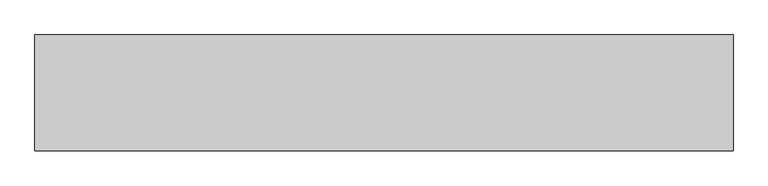
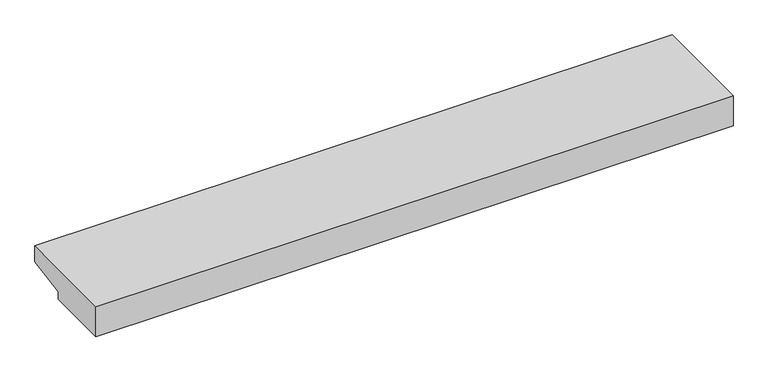
"""IFC4 building model written with IfcOpenShell, lengths in millimetres: plate geometry, 린텔1 : 창대석."""

from ifc_helpers import new_model, si_unit, frame, origin, place, context, project, spatial, polyline, outline, extrude, source, transform, mapped, element, save


def plate_352e0ffc(model_context):
    return source(origin(), model_context, "Body", "SweptSolid", [
        extrude(outline(polyline([(-195.0, 990.0), (435.0, 990.0), (435.0, 890.0), (195.0, 847.6815246), (195.0, 800.0), (-195.0, 800.0), (-195.0, 990.0)])), frame((-1900.0, 0.0, 0.0), z_axis=(1.0, 0.0, 0.0), x_axis=(0.0, 1.0, 0.0)), (0.0, 0.0, 1.0), 3800.0),
    ])


if __name__ == "__main__":
    model = new_model("IFC4")
    model_context = context("Model", 3, world=origin())
    ifc_project = project(units=[si_unit("LENGTHUNIT", "METRE", prefix="MILLI")], contexts=[model_context])
    site = spatial("IfcSite", under=ifc_project)
    building = spatial("IfcBuilding", under=site)
    placement = place(None, origin())
    plate_shape = plate_352e0ffc(model_context)
    element("IfcPlate", 1, ObjectType="린텔1 : 창대석", at=placement, inside=building, context=model_context, shape_type="MappedRepresentation", body=[
        mapped(plate_shape, transform((0.0, 0.0, 0.0), x_axis=(1.0, 0.0, 0.0), y_axis=(0.0, 1.0, 0.0), z_axis=(0.0, 0.0, 1.0))),
    ])
    save(model, "model.ifc")

# Revit data of these elements
# Type "린텔1 : 창대석"
#   Description = "THK.30 GRANITE COUNTER(TYP.)"
#   Type Mark = "200"
#   Description = "THK.30 GRANITE COUNTER(TYP.)"
#   Width = 3800 mm
#   Height = 190 mm
#   두께 = 190 mm
#   돌출부두께 = 190 mm
#   돌출길이 = 240 mm
#   Default Sill Height = 800 mm
#   Wall Closure = (empty or 0)
